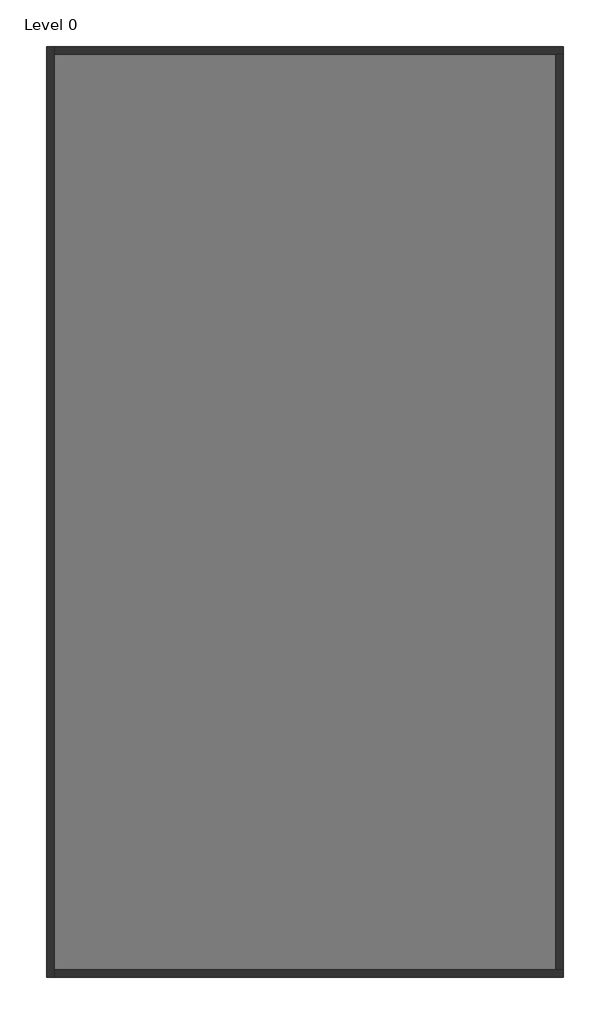
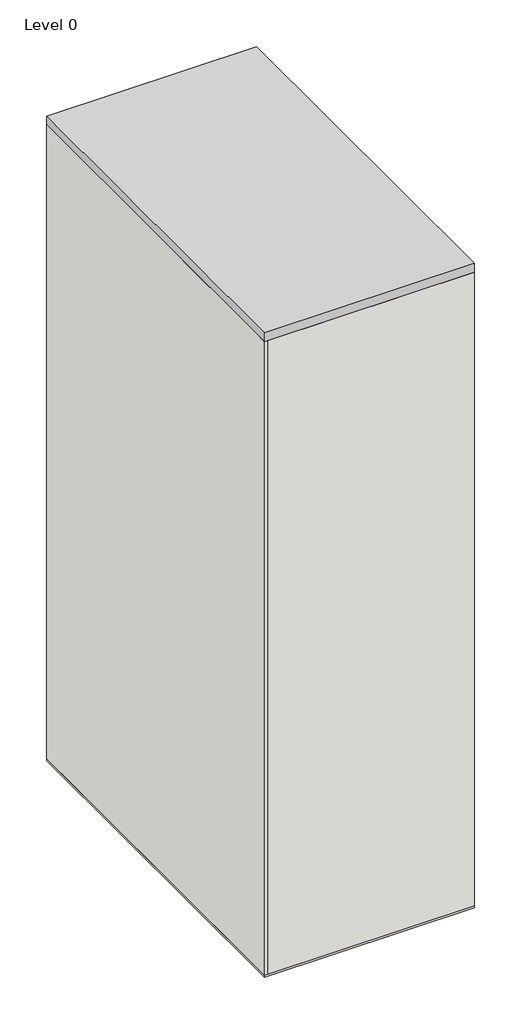
# One storey: 4 walls, 1 proxy, 1 slab.
"""IFC4 building model written with IfcOpenShell, lengths in millimetres."""

from ifc_helpers import new_model, si_unit, frame, origin, origin_with_axes, place, context, project, spatial, polyline, outline, extrude, faceted_brep, element, save

model = new_model("IFC4")

# Units and contexts
model_context = context("Model", 3, world=origin())
ifc_project = project(units=[si_unit("LENGTHUNIT", "METRE", prefix="MILLI")], contexts=[model_context])

# Site, building, storey
site = spatial("IfcSite", under=ifc_project)
building = spatial("IfcBuilding", under=site)
storey = spatial("IfcBuildingStorey", under=building, Name="Level 0", Elevation=100.0)

# Proxy
placement = place(None, origin())
element("IfcBuildingElementProxy", 1, Name="LowUrbanDensityBuilding : LowUrbanDensityBuilding", ObjectType="LowUrbanDensityBuilding : LowUrbanDensityBuilding", at=placement, inside=storey, context=model_context, shape_type="SweptSolid", body=[
    extrude(outline(polyline([(7325.2659446, 3676.2074539), (7325.2659446, -14323.7925461), (-2674.7340554, -14323.7925461), (-2674.7340554, 3676.2074539), (7325.2659446, 3676.2074539)])), origin_with_axes(), (0.0, 0.0, 1.0), 32445.0),
])

# Slab
element("IfcSlab", 2, ObjectType="Floor-Concrete_100Con", at=placement, inside=storey, context=model_context, shape_type="SweptSolid", body=[
    extrude(outline(polyline([(7325.2659446, 3676.2074539), (7325.2659446, -14323.7925461), (-2674.7340554, -14323.7925461), (-2674.7340554, 3676.2074539), (7325.2659446, 3676.2074539)])), origin_with_axes(), (0.0, 0.0, 1.0), 100.0),
])

# Walls
element("IfcWall", 3, ObjectType="Wall-Ext_25Rdr-100Blk-19P", at=placement, inside=storey, context=model_context, shape_type="Brep", body=[
    faceted_brep([(-2674.7340554, 3676.2074539, 100.0), (-2674.7340554, -14323.7925461, 100.0), (-2674.7340554, -14323.7925461, 32000.0), (-2674.7340554, 3676.2074539, 32000.0), (-2530.4340554, 3676.2074539, 100.0), (-2530.4340554, 3676.2074539, 32000.0), (-2530.4340554, 3531.9074539, 32000.0), (-2530.4340554, -14179.4925461, 32000.0), (-2530.4340554, -14323.7925461, 32000.0), (-2530.4340554, -14323.7925461, 100.0), (-2530.4340554, -14179.4925461, 100.0), (-2530.4340554, 3531.9074539, 100.0)], [[[0, 1, 2, 3]], [[4, 5, 6, 7, 8, 9, 10, 11]], [[1, 0, 4, 11, 10, 9]], [[3, 2, 8, 7, 6, 5]], [[2, 1, 9, 8]], [[0, 3, 5, 4]]]),
])
element("IfcWall", 4, ObjectType="Wall-Ext_25Rdr-100Blk-19P", at=placement, inside=storey, context=model_context, shape_type="Brep", body=[
    faceted_brep([(-2530.4340554, -14323.7925461, 100.0), (7325.2659446, -14323.7925461, 100.0), (7325.2659446, -14323.7925461, 32000.0), (-2530.4340554, -14323.7925461, 32000.0), (-2530.4340554, -14179.4925461, 100.0), (-2530.4340554, -14179.4925461, 32000.0), (7180.9659446, -14179.4925461, 32000.0), (7325.2659446, -14179.4925461, 32000.0), (7325.2659446, -14179.4925461, 100.0), (7180.9659446, -14179.4925461, 100.0)], [[[0, 1, 2, 3]], [[4, 5, 6, 7, 8, 9]], [[1, 0, 4, 9, 8]], [[3, 2, 7, 6, 5]], [[0, 3, 5, 4]], [[2, 1, 8, 7]]]),
])
element("IfcWall", 5, ObjectType="Wall-Ext_25Rdr-100Blk-19P", at=placement, inside=storey, context=model_context, shape_type="Brep", body=[
    faceted_brep([(7325.2659446, 3676.2074539, 100.0), (-2530.4340554, 3676.2074539, 100.0), (-2530.4340554, 3676.2074539, 32000.0), (7325.2659446, 3676.2074539, 32000.0), (7325.2659446, 3531.9074539, 100.0), (7325.2659446, 3531.9074539, 32000.0), (7180.9659446, 3531.9074539, 32000.0), (-2530.4340554, 3531.9074539, 32000.0), (-2530.4340554, 3531.9074539, 100.0), (7180.9659446, 3531.9074539, 100.0)], [[[0, 1, 2, 3]], [[4, 5, 6, 7, 8, 9]], [[1, 0, 4, 9, 8]], [[3, 2, 7, 6, 5]], [[2, 1, 8, 7]], [[0, 3, 5, 4]]]),
])
element("IfcWall", 6, ObjectType="Wall-Ext_25Rdr-100Blk-19P", at=placement, inside=storey, context=model_context, shape_type="SweptSolid", body=[
    extrude(outline(polyline([(7325.2659446, 3531.9074539), (7325.2659446, -14179.4925461), (7180.9659446, -14179.4925461), (7180.9659446, 3531.9074539), (7325.2659446, 3531.9074539)])), frame((0.0, 0.0, 100.0), z_axis=(0.0, 0.0, 1.0), x_axis=(1.0, 0.0, 0.0)), (0.0, 0.0, 1.0), 31900.0),
])

save(model, "model.ifc")

# Revit data of these elements
# Project information
#   Project Issue Date = "Issue Date"
#   Project Status = "Project Status"
#   Client Name = "Owner"
#   Project Address = "Enter address here"
#   Project Name = "Project Name"
#   Project Number = "Project Number"
# Type "Floor-Concrete_100Con"
#   Keynote = "E60/130"
#   Function = 0
#   Layers, outside or top first: 100 mm "Concrete" (function 1)
# Type "Wall-Ext_25Rdr-100Blk-19P"
#   Keynote = "F10"
#   Layers, outside or top first: 25.3 mm "Render, Beige, Smooth" (function 5); 100 mm "Concrete Masonry Units _Low Density" (function 1); 19 mm "Plaster" (function 5)
# Element 1 (IfcBuildingElementProxy, "LowUrbanDensityBuilding : LowUrbanDensityBuilding")
#   Phase Created = New Construction
#   Materials on its faces: "Default Form"
# Element 2 (IfcSlab, "Floor-Concrete_100Con")
#   Height Offset From Level = 0 mm
#   Phase Created = New Construction
#   Materials on its faces: "Concrete"
# Element 3 (IfcWall, "Wall-Ext_25Rdr-100Blk-19P")
#   Top Offset = 0 mm
#   Base Offset = 0 mm
#   wall height = 31900 mm
#   Phase Created = New Construction
#   Base Constraint = Level 0
#   Top Constraint = Level 8
#   Materials on its faces: "Render, Beige, Smooth", "Default Wall", "Plaster"
# Elements 4, 5, 6 (IfcWall, "Wall-Ext_25Rdr-100Blk-19P")
#   Top Offset = 0 mm
#   Base Offset = 0 mm
#   wall height = 31900 mm
#   Phase Created = New Construction
#   Base Constraint = Level 0
#   Top Constraint = Level 8
#   Materials on its faces: "Default Wall", "Render, Beige, Smooth", "Plaster"
# Materials
#   "Concrete": class "Concrete", colour RGB 120 120 120, transparency 0, Description = "Portland Cement Concrete", Cost = 0
#   "Render, Beige, Smooth": class "Generic", colour RGB 213 198 180, transparency 0, Description = "physical material", Cost = 0
#   "Concrete Masonry Units _Low Density": class "Masonry", colour RGB 181 181 181, transparency 0, Description = "Concrete masonry units", Cost = 0
#   "Plaster": class "Generic", colour RGB 249 249 249, transparency 0, Description = "Plaster", Cost = 0
#   "Default Form": class "Generic", colour RGB 185 189 196, transparency 0.5, Cost = 0
#   "Default Wall": class "Miscellaneous", colour RGB 128 128 128, transparency 0, Comments = "Rendering appearance not upgraded Rendering appearance not upgraded ", Cost = 0
